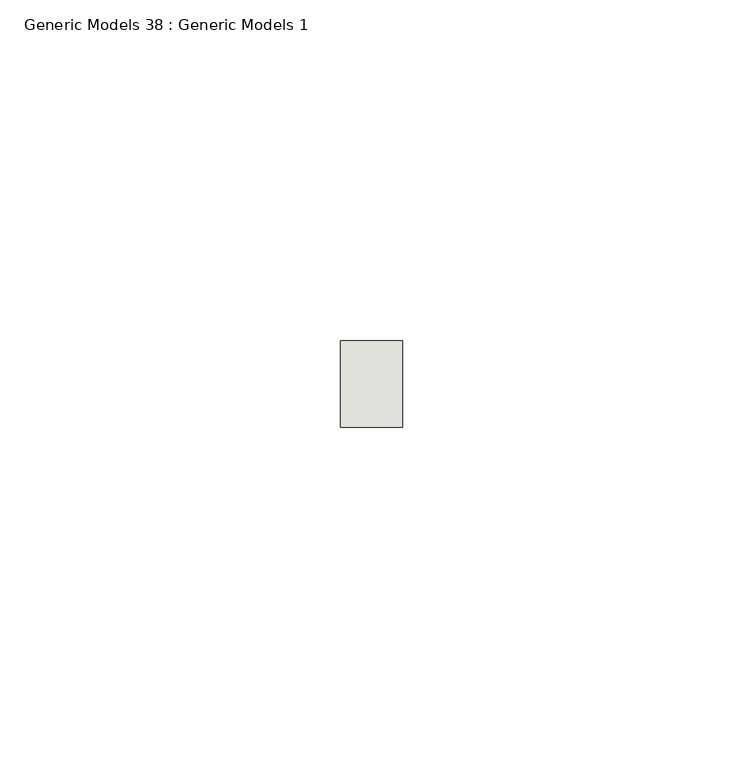
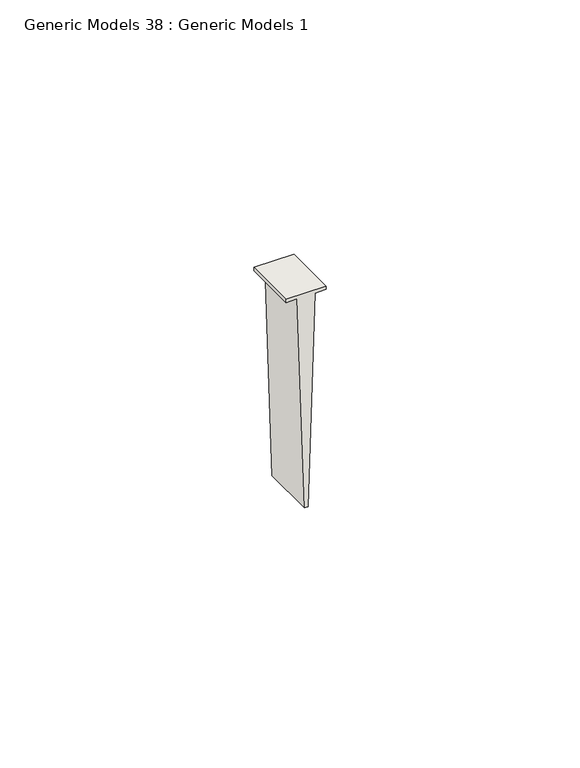
"""IFC4 building model written with IfcOpenShell, lengths in millimetres: wall geometry, Generic Models 38 : Generic Models 1."""

from ifc_helpers import new_model, si_unit, frame, origin, place, context, project, spatial, polyline, outline, extrude, source, transform, mapped, element, save


def generic_models_38_generic_models_1_6cd63f98(model_context):
    return source(origin(), model_context, "Body", "SweptSolid", [
        extrude(outline(polyline([(2.38125, 49733.4159), (1.5875, 49733.4159), (1.5875, 49735.9657636), (-49.2125, 49737.5631527), (-49.2125, 49738.3618473), (1.5875, 49739.9592364), (1.5875, 49742.5091), (2.38125, 49742.5091), (2.38125, 49733.4159)])), frame((0.0, 565.15, 0.0), z_axis=(0.0, 1.0, 0.0), x_axis=(0.0, 0.0, 1.0)), (0.0, 0.0, 1.0), 12.7),
    ])


if __name__ == "__main__":
    model = new_model("IFC4")
    model_context = context("Model", 3, world=origin())
    ifc_project = project(units=[si_unit("LENGTHUNIT", "METRE", prefix="MILLI")], contexts=[model_context])
    site = spatial("IfcSite", under=ifc_project)
    building = spatial("IfcBuilding", under=site)
    placement = place(None, origin())
    generic_models_38_generic_models_1_shape = generic_models_38_generic_models_1_6cd63f98(model_context)
    element("IfcWall", 1, ObjectType="Generic Models 38 : Generic Models 1", at=placement, inside=building, context=model_context, shape_type="MappedRepresentation", body=[
        mapped(generic_models_38_generic_models_1_shape, transform((0.0, 0.0, 0.0), x_axis=(1.0, 0.0, 0.0), y_axis=(0.0, 1.0, 0.0), z_axis=(0.0, 0.0, 1.0))),
    ])
    save(model, "model.ifc")

# Revit data of these elements
# Element 1 (IfcWall, "Generic Models 38 : Generic Models 1")
#   Materials on its faces: "METAL RUNNER CHANNEL; FASTEN @ 24\" O.C."
# Materials
#   "METAL RUNNER CHANNEL; FASTEN @ 24\" O.C.": class "Unassigned", colour RGB 210 209 208, transparency 0, Keynote = "M05121300.02", Cost = 0
